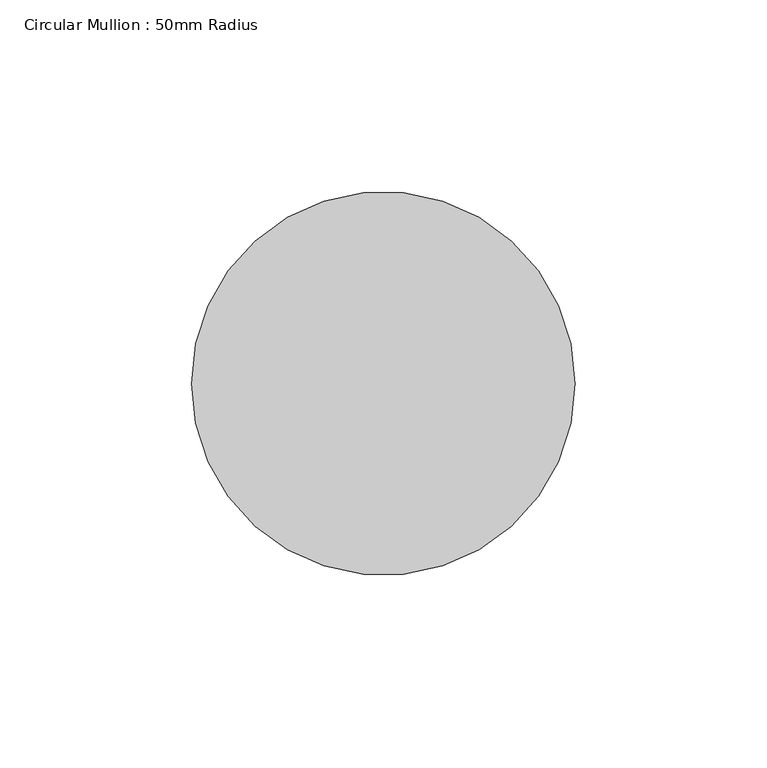
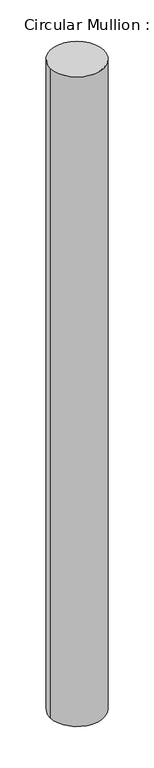
"""IFC4 building model written with IfcOpenShell, lengths in millimetres: member geometry, Circular Mullion : 50mm Radius."""

from ifc_helpers import new_model, si_unit, point, frame, origin, origin_2d, place, context, project, spatial, circle_curve, trimmed, segment, composite_curve, outline, extrude, source, transform, mapped, element, save


def circular_mullion_50mm_radius_edb736c1(model_context):
    return source(origin(), model_context, "Body", "SweptSolid", [
        extrude(outline(composite_curve([segment(trimmed(circle_curve(origin_2d(), 50.0), [point((50.0, 0.0))], [point((-50.0, 0.0))], False, "CARTESIAN"), True, "CONTINUOUS"), segment(trimmed(circle_curve(origin_2d(), 50.0), [point((-50.0, 0.0))], [point((50.0, 0.0))], False, "CARTESIAN"), True, "CONTINUOUS")], self_intersect=False)), frame((0.0, 0.0, -1280.3597493), z_axis=(0.0, 0.0, 1.0), x_axis=(1.0, 0.0, 0.0)), (0.0, 0.0, 1.0), 1280.3597493),
    ])


if __name__ == "__main__":
    model = new_model("IFC4")
    model_context = context("Model", 3, world=origin())
    ifc_project = project(units=[si_unit("LENGTHUNIT", "METRE", prefix="MILLI")], contexts=[model_context])
    site = spatial("IfcSite", under=ifc_project)
    building = spatial("IfcBuilding", under=site)
    placement = place(None, origin())
    circular_mullion_50mm_radius_shape = circular_mullion_50mm_radius_edb736c1(model_context)
    element("IfcMember", 1, ObjectType="Circular Mullion : 50mm Radius", at=placement, inside=building, context=model_context, shape_type="MappedRepresentation", body=[
        mapped(circular_mullion_50mm_radius_shape, transform((0.0, 0.0, 0.0), x_axis=(1.0, 0.0, 0.0), y_axis=(0.0, 1.0, 0.0), z_axis=(0.0, 0.0, 1.0))),
    ])
    save(model, "model.ifc")

# Revit data of these elements
# Type "Circular Mullion : 50mm Radius"
#   built-in parameter 1007350 = 0.164042 (stored number, unit not read)
# Element 1 (IfcMember, "Circular Mullion : 50mm Radius")
#   Materials on its faces: "Aluminium"
# Materials
#   "Aluminium": class "Metal", colour RGB 247 247 247, transparency 0, Description = "Aluminium 6061", Cost = 0
